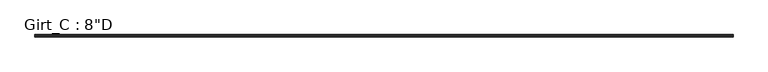
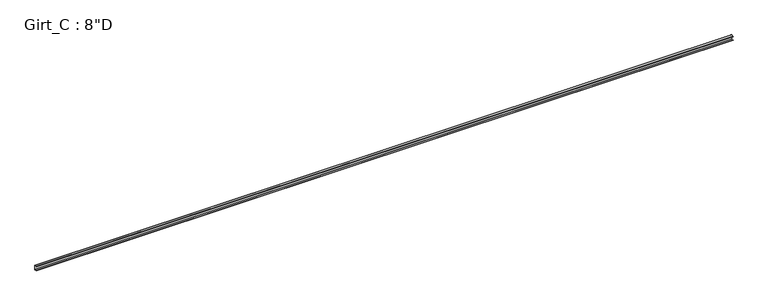
"""IFC4 building model written with IfcOpenShell, lengths in millimetres: beam geometry."""

import ifcopenshell
import ifcopenshell.guid

model = None  # the IFC model being written
_history = None  # IfcOwnerHistory: only IFC2X3 demands one
_inside = {}  # id of a spatial element -> (the spatial element, [elements in it])
_under = {}  # id of a project, library or spatial element -> (it, [spatial elements below it])
_declared = {}  # id of a project -> (the project, [libraries it declares])
_typed = {}  # id of a type object -> (the type object, [elements of that type])
_made_of = {}  # id of a material, layer set ... -> (it, [elements and type objects made of it])


def new_model(schema):
    """Start an empty IFC model of exactly this schema.

    Asked for "IFC4X3", IfcOpenShell would pick the latest addendum, in which some entities
    have other attributes; the version numbers below select the first issue.
    IFC2X3 requires an IfcOwnerHistory on every rooted entity: one is made here for all.
    """
    global model, _history
    if schema == "IFC4X3":
        model = ifcopenshell.file(schema_version=(4, 3, 0, 0))
    else:
        model = ifcopenshell.file(schema=schema)
    _inside.clear()
    _under.clear()
    _declared.clear()
    _typed.clear()
    _made_of.clear()
    _history = None
    if model.schema == "IFC2X3":
        org = make("IfcOrganization", Name="unknown")
        user = make(
            "IfcPersonAndOrganization",
            ThePerson=make("IfcPerson", FamilyName="unknown"),
            TheOrganization=org,
        )
        app = make(
            "IfcApplication",
            ApplicationDeveloper=org,
            Version="unknown",
            ApplicationFullName="unknown",
            ApplicationIdentifier="unknown",
        )
        _history = make(
            "IfcOwnerHistory",
            OwningUser=user,
            OwningApplication=app,
            ChangeAction="ADDED",
            CreationDate=0,
        )
    return model


def make(cls, **values):
    """One entity of the class cls with the attributes given. An attribute that is None is left unset."""
    return model.create_entity(
        cls, **{name: value for name, value in values.items() if value is not None}
    )


def rooted(cls, **values):
    """An entity with a GlobalId (a new one), such as an element, a storey or a relation."""
    return make(cls, GlobalId=ifcopenshell.guid.new(), OwnerHistory=_history, **values)


def si_unit(unit_type, name, prefix=None):
    """IfcSIUnit, for example si_unit("LENGTHUNIT", "METRE", prefix="MILLI")."""
    return make("IfcSIUnit", UnitType=unit_type, Prefix=prefix, Name=name)


def assignment(units):
    """IfcUnitAssignment: the units of a project."""
    return None if units is None else make("IfcUnitAssignment", Units=units)


def point(xyz):
    """IfcCartesianPoint."""
    return None if xyz is None else make("IfcCartesianPoint", Coordinates=xyz)


def direction(xyz):
    """IfcDirection."""
    return None if xyz is None else make("IfcDirection", DirectionRatios=xyz)


def frame(location, z_axis=None, x_axis=None):
    """IfcAxis2Placement3D, a coordinate frame: its origin and axes. An axis left out is left unset."""
    return make(
        "IfcAxis2Placement3D",
        Location=point(location),
        Axis=direction(z_axis),
        RefDirection=direction(x_axis),
    )


def frame_2d(location, x_axis=None):
    """IfcAxis2Placement2D, a coordinate frame in the plane: its origin and x axis."""
    return make(
        "IfcAxis2Placement2D", Location=point(location), RefDirection=direction(x_axis)
    )


def origin():
    """The frame at (0, 0, 0) with its axes left unset."""
    return frame((0.0, 0.0, 0.0))


def place(relative_to, where):
    """IfcLocalPlacement: puts the frame where relative to a parent placement (None: the world)."""
    return make(
        "IfcLocalPlacement", PlacementRelTo=relative_to, RelativePlacement=where
    )


def context(
    kind, dimensions, precision=None, world=None, true_north=None, identifier=None
):
    """IfcGeometricRepresentationContext, for example the 3D "Model" context."""
    return make(
        "IfcGeometricRepresentationContext",
        ContextIdentifier=identifier,
        ContextType=kind,
        CoordinateSpaceDimension=dimensions,
        Precision=precision,
        WorldCoordinateSystem=world,
        TrueNorth=true_north,
    )


def project(units=None, contexts=None):
    """IfcProject with its units and contexts."""
    return rooted(
        "IfcProject",
        Name="project",
        RepresentationContexts=contexts,
        UnitsInContext=assignment(units),
    )


def spatial(cls, under=None, at=None, **own):
    """A site, building, storey or space (cls), placed at a placement, below another one or the project."""
    s = rooted(cls, ObjectPlacement=at, **own)
    if under is not None:
        _under.setdefault(under.id(), (under, []))[1].append(s)
    return s


def polyline(points):
    """IfcPolyline through the points."""
    return make("IfcPolyline", Points=[point(p) for p in points])


def circle_curve(where, radius):
    """IfcCircle in the frame where."""
    return make("IfcCircle", Position=where, Radius=radius)


def trimmed(basis, trim1, trim2, sense, master):
    """IfcTrimmedCurve: the piece of a basis curve between two trims."""
    return make(
        "IfcTrimmedCurve",
        BasisCurve=basis,
        Trim1=trim1,
        Trim2=trim2,
        SenseAgreement=sense,
        MasterRepresentation=master,
    )


def segment(curve, same_sense, transition):
    """IfcCompositeCurveSegment."""
    return make(
        "IfcCompositeCurveSegment",
        Transition=transition,
        SameSense=same_sense,
        ParentCurve=curve,
    )


def composite_curve(segments, self_intersect=None):
    """IfcCompositeCurve: segments joined end to end."""
    return make("IfcCompositeCurve", Segments=segments, SelfIntersect=self_intersect)


def outline(outer, holes=None, kind="AREA"):
    """IfcArbitraryClosedProfileDef: a profile drawn as a closed curve; with holes, ...WithVoids."""
    if holes is None:
        return make("IfcArbitraryClosedProfileDef", ProfileType=kind, OuterCurve=outer)
    return make(
        "IfcArbitraryProfileDefWithVoids",
        ProfileType=kind,
        OuterCurve=outer,
        InnerCurves=holes,
    )


def extrude(swept, where, along, depth):
    """IfcExtrudedAreaSolid: the profile swept, set in the frame where, extruded along a direction by depth."""
    return make(
        "IfcExtrudedAreaSolid",
        SweptArea=swept,
        Position=where,
        ExtrudedDirection=direction(along),
        Depth=depth,
    )


def shape(context_of_items, identifier, shape_type, items):
    """IfcShapeRepresentation: the items that make up one representation, for example the "Body"."""
    return make(
        "IfcShapeRepresentation",
        ContextOfItems=context_of_items,
        RepresentationIdentifier=identifier,
        RepresentationType=shape_type,
        Items=items,
    )


def source(mapping_origin, context_of_items, identifier, shape_type, items):
    """IfcRepresentationMap: a shape defined once, which mapped items show again and again."""
    return make(
        "IfcRepresentationMap",
        MappingOrigin=mapping_origin,
        MappedRepresentation=shape(context_of_items, identifier, shape_type, items),
    )


def transform(
    local_origin,
    x_axis=None,
    y_axis=None,
    z_axis=None,
    scale=None,
    scale2=None,
    scale3=None,
    uniform=True,
):
    """IfcCartesianTransformationOperator3D, or its non-uniform kind. x_axis, y_axis, z_axis: its Axis1, 2, 3."""
    if uniform:
        return make(
            "IfcCartesianTransformationOperator3D",
            Axis1=direction(x_axis),
            Axis2=direction(y_axis),
            LocalOrigin=point(local_origin),
            Scale=scale,
            Axis3=direction(z_axis),
        )
    return make(
        "IfcCartesianTransformationOperator3DnonUniform",
        Axis1=direction(x_axis),
        Axis2=direction(y_axis),
        LocalOrigin=point(local_origin),
        Scale=scale,
        Axis3=direction(z_axis),
        Scale2=scale2,
        Scale3=scale3,
    )


def mapped(mapping_source, mapping_target):
    """IfcMappedItem: shows the shape of a source again, moved by a transform."""
    return make(
        "IfcMappedItem", MappingSource=mapping_source, MappingTarget=mapping_target
    )


def made_of(thing, what):
    """Note that an element or type object is made of a material, layer set ...; save() writes the relation."""
    if what is not None:
        _made_of.setdefault(what.id(), (what, []))[1].append(thing)
    return thing


def element(
    cls,
    number,
    at=None,
    inside=None,
    cuts=None,
    type_object=None,
    material=None,
    context=None,
    identifier="Body",
    shape_type=None,
    held_by="IfcProductDefinitionShape",
    body=None,
    shapes=None,
    **own,
):
    """One element of the class cls, such as IfcWall. Its Tag is "e" and its number.

    at: its placement. inside: the storey or other place that contains it. cuts: it is an
    opening in that element (IfcRelVoidsElement). A single representation is given by context,
    identifier, shape_type and body (its items); several are given by shapes. held_by: the class
    of the entity that holds the representations. save() writes the other relations.
    """
    e = rooted(cls, Tag="e%d" % number, ObjectPlacement=at, **own)
    if body is not None:
        shapes = [shape(context, identifier, shape_type, body)]
    if shapes is not None:
        e.Representation = make(held_by, Representations=shapes)
    if inside is not None:
        _inside.setdefault(inside.id(), (inside, []))[1].append(e)
    if cuts is not None:
        rooted(
            "IfcRelVoidsElement", RelatingBuildingElement=cuts, RelatedOpeningElement=e
        )
    if type_object is not None:
        _typed.setdefault(type_object.id(), (type_object, []))[1].append(e)
    return made_of(e, material)


def aggregate(whole, parts):
    """IfcRelAggregates: a whole, such as a stair, and the parts it consists of."""
    return rooted("IfcRelAggregates", RelatingObject=whole, RelatedObjects=parts)


def save(model, path):
    """Write the relations noted so far, then the file.

    IfcRelAggregates (storeys below a building ...), IfcRelContainedInSpatialStructure (elements
    in a storey), IfcRelDefinesByType, IfcRelAssociatesMaterial and IfcRelDeclares: one each for
    every whole, place, type object, material and project.
    """
    for whole, parts in _under.values():
        aggregate(whole, parts)
    for where, things in _inside.values():
        rooted(
            "IfcRelContainedInSpatialStructure",
            RelatedElements=things,
            RelatingStructure=where,
        )
    for kind, things in _typed.values():
        rooted("IfcRelDefinesByType", RelatedObjects=things, RelatingType=kind)
    for what, things in _made_of.values():
        rooted("IfcRelAssociatesMaterial", RelatedObjects=things, RelatingMaterial=what)
    for by, libraries in _declared.values():
        rooted("IfcRelDeclares", RelatingContext=by, RelatedDefinitions=libraries)
    model.write(path)


def beam_fb6f6511(model_context):
    return source(origin(), model_context, "Body", "SweptSolid", [
        extrude(outline(composite_curve([segment(polyline([(-87.5109375, 101.6), (-3.3734375, 101.6)]), True, "CONTINUOUS"), segment(trimmed(circle_curve(frame_2d((-3.3734375, 96.8375)), 4.7625), [point((-3.3734375, 101.6))], [point((1.3890625, 96.8375))], False, "CARTESIAN"), True, "CONTINUOUS"), segment(polyline([(1.3890625, 96.8375), (1.3890625, -96.8375)]), True, "CONTINUOUS"), segment(trimmed(circle_curve(frame_2d((-3.3734375, -96.8375)), 4.7625), [point((1.3890625, -96.8375))], [point((-3.3734375, -101.6))], False, "CARTESIAN"), True, "CONTINUOUS"), segment(polyline([(-3.3734375, -101.6), (-87.5109375, -101.6), (-99.7792647, -86.979177), (-97.6510975, -85.1934327), (-86.2154765, -98.821875), (-3.2694106, -98.821875)]), True, "CONTINUOUS"), segment(trimmed(circle_curve(frame_2d((-3.3748024, -96.8389339)), 1.9857399), [point((-3.2694106, -98.821875))], [point((-1.3890625, -96.8389339))], True, "CARTESIAN"), True, "CONTINUOUS"), segment(polyline([(-1.3890625, -96.8389339), (-1.3890625, 96.8381931)]), True, "CONTINUOUS"), segment(trimmed(circle_curve(frame_2d((-3.3741066, 96.8381931)), 1.9850441), [point((-1.3890625, 96.8381931))], [point((-3.3005807, 98.821875))], True, "CARTESIAN"), True, "CONTINUOUS"), segment(polyline([(-3.3005807, 98.821875), (-86.2154765, 98.821875), (-97.6278742, 85.221109), (-99.7560415, 87.0068534), (-87.5109375, 101.6)]), True, "CONTINUOUS")], self_intersect=False)), frame((-15570.2, 0.0, 0.0), z_axis=(1.0, 0.0, 0.0), x_axis=(0.0, 1.0, 0.0)), (0.0, 0.0, 1.0), 31140.4),
    ])


if __name__ == "__main__":
    model = new_model("IFC4")
    model_context = context("Model", 3, world=origin())
    ifc_project = project(units=[si_unit("LENGTHUNIT", "METRE", prefix="MILLI")], contexts=[model_context])
    site = spatial("IfcSite", under=ifc_project)
    building = spatial("IfcBuilding", under=site)
    placement = place(None, origin())
    beam_shape = beam_fb6f6511(model_context)
    element("IfcBeam", 1, ObjectType="Girt_C : 8\"D", at=placement, inside=building, context=model_context, shape_type="MappedRepresentation", body=[
        mapped(beam_shape, transform((0.0, 0.0, 0.0), x_axis=(1.0, 0.0, 0.0), y_axis=(0.0, 1.0, 0.0), z_axis=(0.0, 0.0, 1.0))),
    ])
    save(model, "model.ifc")

# Revit data of these elements
# Type "Girt_C : 8\"D"
#   half leg = 0' - 1 3/4"
#   Web_Thickness = 0' - 0 7/64"
#   Length [instance default] = 10' - 0"
#   Leg_1 = 0' - 3 1/2"
#   Height = 0' - 8"
#   Structural Material [instance default] = none
# Element 1 (IfcBeam, "Girt_C : 8\"D")
#   Structural Material = CEE' SECTION (8.0x3.5C - SEE STRUCT. DWGS)
#   Materials on its faces: "CEE' SECTION (8.0x3.5C - SEE STRUCT. DWGS)"
# Materials
#   "CEE' SECTION (8.0x3.5C - SEE STRUCT. DWGS)": class "Metal", colour RGB 137 146 153, transparency 0, Description = "Steel, mill finish", Cost = 0
